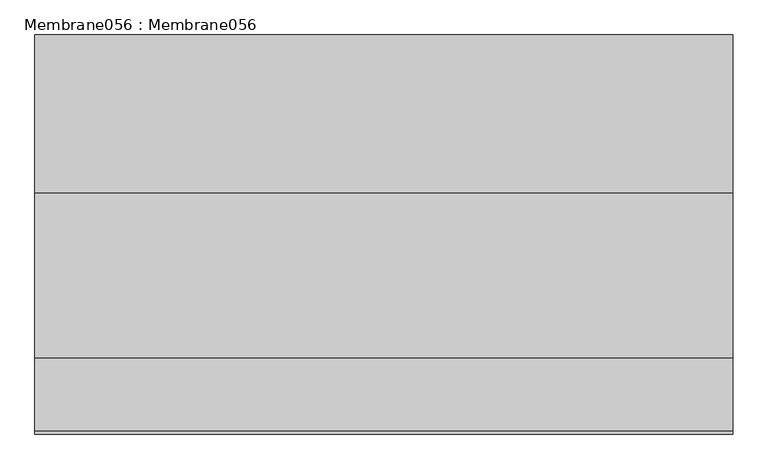
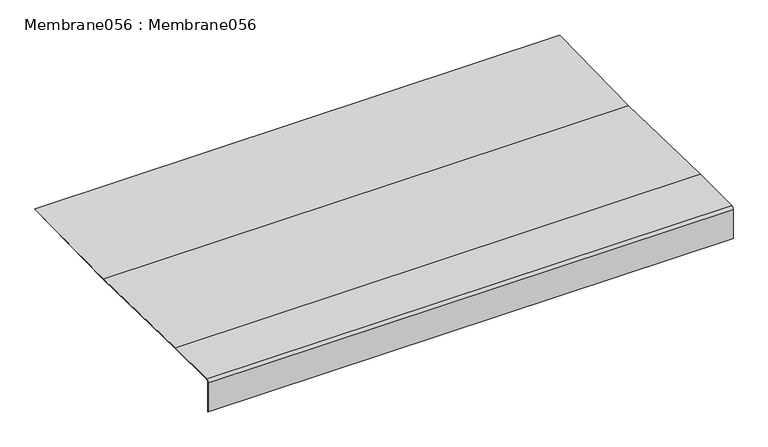
"""IFC4 building model written with IfcOpenShell, lengths in millimetres: proxy geometry, Membrane056 : Membrane056."""

from ifc_helpers import new_model, si_unit, point, frame, frame_2d, origin, place, context, project, spatial, polyline, circle_curve, trimmed, segment, composite_curve, outline, extrude, source, transform, mapped, element, save


def membrane056_membrane056_fd08afe1(model_context):
    return source(origin(), model_context, "Body", "SweptSolid", [
        extrude(outline(composite_curve([segment(polyline([(-5564.3684261, 40101.8965244), (-5566.3684261, 40101.8965244), (-5566.3684261, 40218.6165225)]), True, "CONTINUOUS"), segment(trimmed(circle_curve(frame_2d((-5556.3684261, 40218.6165225)), 10.0), [point((-5566.3684261, 40218.6165225))], [point((-5556.3684261, 40228.6165225))], False, "CARTESIAN"), True, "CONTINUOUS"), segment(polyline([(-5556.3684261, 40228.6165225), (-5348.0337978, 40228.6165225), (-4874.4404297, 40217.78125), (-4422.9526514, 40227.5556977), (-4422.9093627, 40225.5561663), (-4874.4416589, 40215.7807547), (-5348.0566737, 40226.6165225), (-5556.3684261, 40226.6165225)]), True, "CONTINUOUS"), segment(trimmed(circle_curve(frame_2d((-5556.3684261, 40218.6165225)), 8.0), [point((-5556.3684261, 40226.6165225))], [point((-5564.3684261, 40218.6165225))], True, "CARTESIAN"), True, "CONTINUOUS"), segment(polyline([(-5564.3684261, 40218.6165225), (-5564.3684261, 40101.8965244)]), True, "CONTINUOUS")], self_intersect=False)), frame((12383.0178845, 0.0, 0.0), z_axis=(1.0, 0.0, 0.0), x_axis=(0.0, 1.0, 0.0)), (0.0, 0.0, 1.0), 2000.0),
    ])


if __name__ == "__main__":
    model = new_model("IFC4")
    model_context = context("Model", 3, world=origin())
    ifc_project = project(units=[si_unit("LENGTHUNIT", "METRE", prefix="MILLI")], contexts=[model_context])
    site = spatial("IfcSite", under=ifc_project)
    building = spatial("IfcBuilding", under=site)
    placement = place(None, origin())
    membrane056_membrane056_shape = membrane056_membrane056_fd08afe1(model_context)
    element("IfcBuildingElementProxy", 1, Name="Membrane056 : Membrane056", ObjectType="Membrane056 : Membrane056", at=placement, inside=building, context=model_context, shape_type="MappedRepresentation", body=[
        mapped(membrane056_membrane056_shape, transform((0.0, 0.0, 0.0), x_axis=(1.0, 0.0, 0.0), y_axis=(0.0, 1.0, 0.0), z_axis=(0.0, 0.0, 1.0))),
    ])
    save(model, "model.ifc")

# Revit data of these elements
# Type "Membrane056 : Membrane056"
#   NameOverride = "Membrane056"
# Element 1 (IfcBuildingElementProxy, "Membrane056 : Membrane056")
#   Materials on its faces: "THREE PLY BUILT UP ROOF MEMBRANE"
# Materials
#   "THREE PLY BUILT UP ROOF MEMBRANE": class "Unassigned", colour RGB 63 63 63, transparency 0
